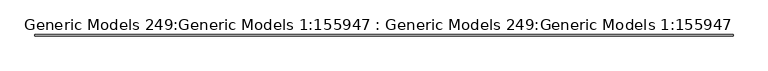
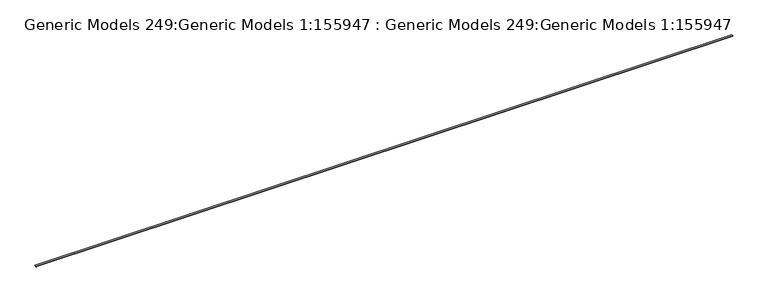
"""IFC4 building model written with IfcOpenShell, lengths in millimetres: proxy geometry, Generic Models 249:Generic Models 1:155947 : Generic Models 249:Generic Models 1:155947."""

from ifc_helpers import new_model, si_unit, frame, origin, place, context, project, spatial, polyline, outline, extrude, source, transform, mapped, element, save


def generic_models_249_generic_models_1_155947_generic_models_d061952d(model_context):
    return source(origin(), model_context, "Body", "SweptSolid", [
        extrude(outline(polyline([(11998.8426662, 3044.825), (11994.0928662, 3044.825), (11994.0928662, 3067.05), (12032.1928662, 3067.05), (12032.1928662, 3065.78), (11995.3628662, 3065.78), (11995.3628662, 3046.095), (11997.5726662, 3046.095), (11997.5726662, 3047.8274564), (11998.8426662, 3047.8274564), (11998.8426662, 3044.825)])), frame((-10606.0105468, 0.0, 0.0), z_axis=(1.0, 0.0, 0.0), x_axis=(0.0, 1.0, 0.0)), (0.0, 0.0, 1.0), 19050.0),
    ])


if __name__ == "__main__":
    model = new_model("IFC4")
    model_context = context("Model", 3, world=origin())
    ifc_project = project(units=[si_unit("LENGTHUNIT", "METRE", prefix="MILLI")], contexts=[model_context])
    site = spatial("IfcSite", under=ifc_project)
    building = spatial("IfcBuilding", under=site)
    placement = place(None, origin())
    generic_models_249_generic_models_1_155947_generic_models_shape = generic_models_249_generic_models_1_155947_generic_models_d061952d(model_context)
    element("IfcBuildingElementProxy", 1, Name="Generic Models 249:Generic Models 1:155947 : Generic Models 249:Generic Models 1:155947", ObjectType="Generic Models 249:Generic Models 1:155947 : Generic Models 249:Generic Models 1:155947", at=placement, inside=building, context=model_context, shape_type="MappedRepresentation", body=[
        mapped(generic_models_249_generic_models_1_155947_generic_models_shape, transform((0.0, 0.0, 0.0), x_axis=(1.0, 0.0, 0.0), y_axis=(0.0, 1.0, 0.0), z_axis=(0.0, 0.0, 1.0))),
    ])
    save(model, "model.ifc")

# Revit data of these elements
# Type "Generic Models 249:Generic Models 1:155947 : Generic Models 249:Generic Models 1:155947"
#   NameOverride = "Generic Models 249:Generic Models 1:155947"
#   ObjectTypeOverride = "Generic Models 249:Generic Models 1"
#   Reference = "Generic Models 1"
#   Category = "Generic Models"
#   Tag = "155947"
# Element 1 (IfcBuildingElementProxy, "Generic Models 249:Generic Models 1:155947 : Generic Models 249:Generic Models 1:155947")
#   Materials on its faces: "_CONTINUOUS 16 GA. COPPER  J BEAD 1960"
# Materials
#   "_CONTINUOUS 16 GA. COPPER  J BEAD 1960": class "Unassigned", colour RGB 253 192 103, transparency 0
